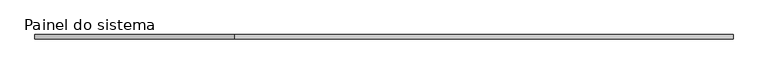
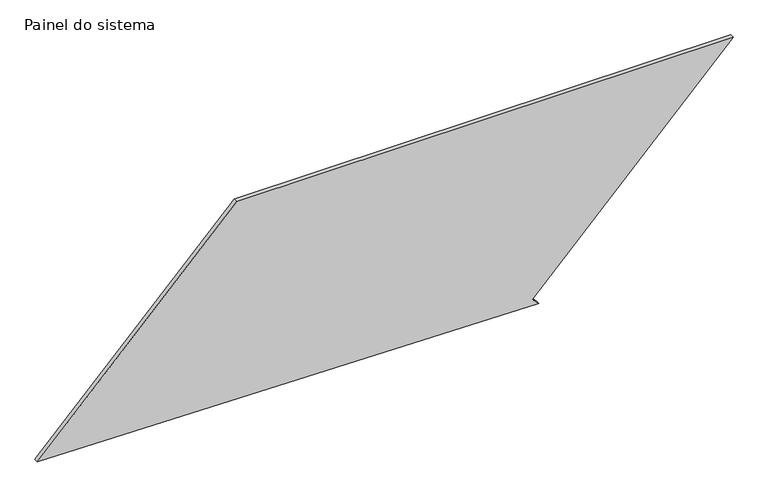
"""IFC4 building model written with IfcOpenShell, lengths in millimetres: plate geometry, Painel do sistema : Envidraçado."""

from ifc_helpers import new_model, si_unit, frame, origin, place, context, project, spatial, polyline, outline, extrude, source, transform, mapped, element, save


def painel_do_sistema_fdae9815(model_context):
    return source(origin(), model_context, "Body", "SweptSolid", [
        extrude(outline(polyline([(0.0, 886.4233209), (34.7865251, 850.5081754), (1233.1195883, 2011.1840593), (1233.1195883, -859.2697134), (43.832324, -2011.1840593), (0.0, 886.4233209)])), frame((0.0, 24.5, 0.0), z_axis=(0.0, 1.0, 0.0), x_axis=(0.0, 0.0, 1.0)), (0.0, 0.0, 1.0), 25.0),
    ])


if __name__ == "__main__":
    model = new_model("IFC4")
    model_context = context("Model", 3, world=origin())
    ifc_project = project(units=[si_unit("LENGTHUNIT", "METRE", prefix="MILLI")], contexts=[model_context])
    site = spatial("IfcSite", under=ifc_project)
    building = spatial("IfcBuilding", under=site)
    placement = place(None, origin())
    painel_do_sistema_shape = painel_do_sistema_fdae9815(model_context)
    element("IfcPlate", 1, ObjectType="Painel do sistema : Envidraçado", at=placement, inside=building, context=model_context, shape_type="MappedRepresentation", body=[
        mapped(painel_do_sistema_shape, transform((0.0, 0.0, 0.0), x_axis=(1.0, 0.0, 0.0), y_axis=(0.0, 1.0, 0.0), z_axis=(0.0, 0.0, 1.0))),
    ])
    save(model, "model.ifc")

# Revit data of these elements
# Type "Painel do sistema : Envidraçado"
#   Construction Type Id = "GSP4R"
#   Analytic Construction = "Vidraça única Pilkington 1/8 pol"
#   Visual Light Transmittance = 0.9
#   Solar Heat Gain Coefficient = 0.86
#   Heat Transfer Coefficient (U) = 6.7069 W/(m²·K)
# Element 1 (IfcPlate, "Painel do sistema : Envidraçado")
#   Materials on its faces: "Vidro"
# Materials
#   "Vidro": class "Vidro", colour RGB 0 128 192, transparency 0.9, Description = "Vidro de sílica", Cost = 0
